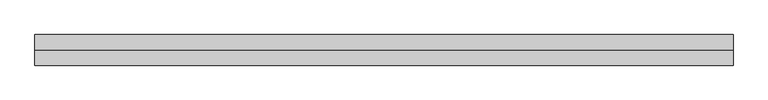
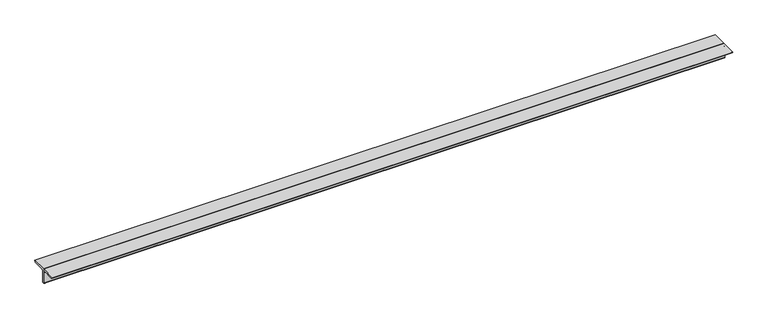
"""IFC4 building model written with IfcOpenShell, lengths in millimetres: member geometry, 0123_Steel Framing_2Ls-KSD3502 : H_SB_AR_S03_2Ls-130x130x12_HBR1."""

from ifc_helpers import new_model, si_unit, point, frame, frame_2d, origin, place, context, project, spatial, polyline, circle_curve, trimmed, segment, composite_curve, outline, extrude, source, transform, mapped, element, save


def member_e3b25103(model_context):
    return source(origin(), model_context, "Body", "SweptSolid", [
        extrude(outline(composite_curve([segment(polyline([(0.0, 36.4), (130.0, 36.4)]), True, "CONTINUOUS"), segment(trimmed(circle_curve(frame_2d((118.0, 36.4)), 12.0), [point((130.0, 36.4))], [point((118.0, 24.4))], False, "CARTESIAN"), True, "CONTINUOUS"), segment(polyline([(118.0, 24.4), (24.0, 24.4)]), True, "CONTINUOUS"), segment(trimmed(circle_curve(frame_2d((24.0, 12.4)), 12.0), [point((24.0, 24.4))], [point((12.0, 12.4))], True, "CARTESIAN"), True, "CONTINUOUS"), segment(polyline([(12.0, 12.4), (12.0, -81.6)]), True, "CONTINUOUS"), segment(trimmed(circle_curve(frame_2d((0.0, -81.6)), 12.0), [point((12.0, -81.6))], [point((0.0, -93.6))], False, "CARTESIAN"), True, "CONTINUOUS"), segment(polyline([(0.0, -93.6), (0.0, 36.4)]), True, "CONTINUOUS")], self_intersect=False)), frame((-2965.840786, 0.0, 0.0), z_axis=(1.0, 0.0, 0.0), x_axis=(0.0, 1.0, 0.0)), (0.0, 0.0, 1.0), 5929.4021426),
        extrude(outline(composite_curve([segment(polyline([(0.0, 36.4), (0.0, -93.6)]), True, "CONTINUOUS"), segment(trimmed(circle_curve(frame_2d((0.0, -81.6)), 12.0), [point((0.0, -93.6))], [point((-12.0, -81.6))], False, "CARTESIAN"), True, "CONTINUOUS"), segment(polyline([(-12.0, -81.6), (-12.0, 12.4)]), True, "CONTINUOUS"), segment(trimmed(circle_curve(frame_2d((-24.0, 12.4)), 12.0), [point((-12.0, 12.4))], [point((-24.0, 24.4))], True, "CARTESIAN"), True, "CONTINUOUS"), segment(polyline([(-24.0, 24.4), (-118.0, 24.4)]), True, "CONTINUOUS"), segment(trimmed(circle_curve(frame_2d((-118.0, 36.4)), 12.0), [point((-118.0, 24.4))], [point((-130.0, 36.4))], False, "CARTESIAN"), True, "CONTINUOUS"), segment(polyline([(-130.0, 36.4), (0.0, 36.4)]), True, "CONTINUOUS")], self_intersect=False)), frame((-2965.840786, 0.0, 0.0), z_axis=(1.0, 0.0, 0.0), x_axis=(0.0, 1.0, 0.0)), (0.0, 0.0, 1.0), 5929.4021426),
    ])


if __name__ == "__main__":
    model = new_model("IFC4")
    model_context = context("Model", 3, world=origin())
    ifc_project = project(units=[si_unit("LENGTHUNIT", "METRE", prefix="MILLI")], contexts=[model_context])
    site = spatial("IfcSite", under=ifc_project)
    building = spatial("IfcBuilding", under=site)
    placement = place(None, origin())
    member_shape = member_e3b25103(model_context)
    element("IfcMember", 1, ObjectType="0123_Steel Framing_2Ls-KSD3502 : H_SB_AR_S03_2Ls-130x130x12_HBR1", at=placement, inside=building, context=model_context, shape_type="MappedRepresentation", body=[
        mapped(member_shape, transform((0.0, 0.0, 0.0), x_axis=(1.0, 0.0, 0.0), y_axis=(0.0, 1.0, 0.0), z_axis=(0.0, 0.0, 1.0))),
    ])
    save(model, "model.ifc")

# Revit data of these elements
# Type "0123_Steel Framing_2Ls-KSD3502 : H_SB_AR_S03_2Ls-130x130x12_HBR1"
#   Type Mark = "HBR1"
#   Assembly Code = "B10"
#   Legs = "SLBB"
#   W = 8.97
#   Perimeter = 1.04 m²/m
#   Nominal Weight = 46.80 kgf/m
#   Length [instance default] = 1000 mm
#   Space = 0 mm
#   b = 130 mm
#   d = 130 mm
#   t = 12 mm
#   y = 36.4 mm
#   A = 0.005952 m²
#   Structural Material [instance default] = Steel ASTM A36
# Element 1 (IfcMember, "0123_Steel Framing_2Ls-KSD3502 : H_SB_AR_S03_2Ls-130x130x12_HBR1")
#   Materials on its faces: "Steel ASTM A36"
# Materials
#   "Steel ASTM A36": class "Metal", colour RGB 199 199 199, transparency 0, Description = "Structural steel, ASTM A36 Grade B, mill finish", Cost = 0
